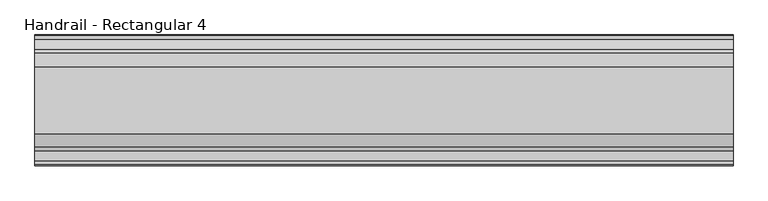
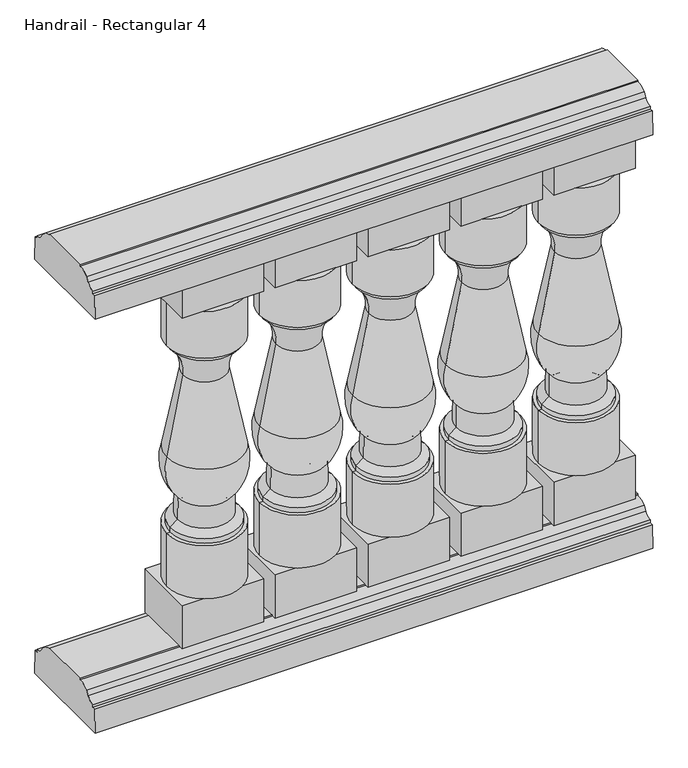
"""IFC4 building model written with IfcOpenShell, lengths in millimetres: railing geometry, Handrail - Rectangular 4."""

from ifc_helpers import new_model, si_unit, point, frame, frame_2d, origin, place, context, project, spatial, polyline, circle_curve, ellipse_curve, trimmed, segment, composite_curve, outline, extrude, source, transform, mapped, element, save
from ifc_brep_helpers import plane_surface, cylinder_surface, revolved_surface, advanced_brep


def handrail_rectangular_4_919d9a96(model_context):
    return source(origin(), model_context, "Body", "SolidModel", [
        extrude(outline(composite_curve([segment(trimmed(circle_curve(frame_2d((-1771.1852268, 1054.89375)), 19.84375), [point((-1771.1852268, 1035.05))], [point((-1754.064785, 1044.8605607))], True, "CARTESIAN"), True, "CONTINUOUS"), segment(polyline([(-1754.064785, 1044.8605607), (-1747.604713, 1054.3201059)]), True, "CONTINUOUS"), segment(trimmed(circle_curve(frame_2d((-1723.5602268, 1027.90625)), 35.71875), [point((-1747.604713, 1054.3201059))], [point((-1723.5602268, 1063.625))], False, "CARTESIAN"), True, "CONTINUOUS"), segment(polyline([(-1723.5602268, 1063.625), (-1723.5602268, 1066.8), (-1607.6727268, 1066.8), (-1607.6727268, 1063.625)]), True, "CONTINUOUS"), segment(trimmed(circle_curve(frame_2d((-1607.6727268, 1027.90625)), 35.71875), [point((-1607.6727268, 1063.625))], [point((-1583.6282406, 1054.3201059))], False, "CARTESIAN"), True, "CONTINUOUS"), segment(polyline([(-1583.6282406, 1054.3201059), (-1577.1681686, 1044.8605607)]), True, "CONTINUOUS"), segment(trimmed(circle_curve(frame_2d((-1560.0477268, 1054.89375)), 19.84375), [point((-1577.1681686, 1044.8605607))], [point((-1560.0477268, 1035.05))], True, "CARTESIAN"), True, "CONTINUOUS"), segment(polyline([(-1560.0477268, 1035.05), (-1560.0477268, 1028.7), (-1552.9039768, 1028.7), (-1551.3164768, 974.725), (-1779.9164768, 974.725), (-1778.3289768, 1028.7), (-1771.1852268, 1028.7), (-1771.1852268, 1035.05)]), True, "CONTINUOUS")], self_intersect=False)), frame((13827.6521895, 0.0, 0.0), z_axis=(1.0, 0.0, 0.0), x_axis=(0.0, 1.0, 0.0)), (0.0, 0.0, 1.0), 1219.2),
        extrude(outline(composite_curve([segment(trimmed(circle_curve(frame_2d((-1771.1852268, 99.21875)), 19.84375), [point((-1771.1852268, 79.375))], [point((-1754.064785, 89.1855607))], True, "CARTESIAN"), True, "CONTINUOUS"), segment(polyline([(-1754.064785, 89.1855607), (-1747.604713, 98.6451059)]), True, "CONTINUOUS"), segment(trimmed(circle_curve(frame_2d((-1723.5602268, 72.23125)), 35.71875), [point((-1747.604713, 98.6451059))], [point((-1723.5602268, 107.95))], False, "CARTESIAN"), True, "CONTINUOUS"), segment(polyline([(-1723.5602268, 107.95), (-1723.5602268, 111.125), (-1607.6727268, 111.125), (-1607.6727268, 107.95)]), True, "CONTINUOUS"), segment(trimmed(circle_curve(frame_2d((-1607.6727268, 72.23125)), 35.71875), [point((-1607.6727268, 107.95))], [point((-1583.6282406, 98.6451059))], False, "CARTESIAN"), True, "CONTINUOUS"), segment(polyline([(-1583.6282406, 98.6451059), (-1577.1681686, 89.1855607)]), True, "CONTINUOUS"), segment(trimmed(circle_curve(frame_2d((-1560.0477268, 99.21875)), 19.84375), [point((-1577.1681686, 89.1855607))], [point((-1560.0477268, 79.375))], True, "CARTESIAN"), True, "CONTINUOUS"), segment(polyline([(-1560.0477268, 79.375), (-1560.0477268, 73.025), (-1552.9039768, 73.025), (-1551.3164768, 19.05), (-1779.9164768, 19.05), (-1778.3289768, 73.025), (-1771.1852268, 73.025), (-1771.1852268, 79.375)]), True, "CONTINUOUS")], self_intersect=False)), frame((13827.6521895, 0.0, 0.0), z_axis=(1.0, 0.0, 0.0), x_axis=(0.0, 1.0, 0.0)), (0.0, 0.0, 1.0), 1219.2),
        advanced_brep(
        [(14862.7021895, -1665.6164768, 874.7125), (15027.8021895, -1665.6164768, 874.7125), (14945.2521895, -1665.6164768, 874.7125), (14862.7021895, -1665.6164768, 766.7625), (15027.8021895, -1665.6164768, 766.7625), (14870.6396895, -1665.6164768, 766.7625), (15019.8646895, -1665.6164768, 766.7625), (14870.6396895, -1665.6164768, 755.65), (15019.8646895, -1665.6164768, 755.65), (14898.4209395, -1665.6164768, 687.3875), (14992.0834395, -1665.6164768, 687.3875), (14863.4959395, -1665.6164768, 509.5875), (15027.0084395, -1665.6164768, 509.5875), (14887.3084395, -1665.6164768, 407.9875), (15003.1959395, -1665.6164768, 407.9875), (14886.5146895, -1665.6164768, 357.1875), (15003.9896895, -1665.6164768, 357.1875), (14870.6396895, -1665.6164768, 344.4875), (15019.8646895, -1665.6164768, 344.4875), (14870.6396895, -1665.6164768, 333.375), (15019.8646895, -1665.6164768, 333.375), (14862.7021895, -1665.6164768, 333.375), (15027.8021895, -1665.6164768, 333.375), (14862.7021895, -1665.6164768, 211.1375), (15027.8021895, -1665.6164768, 211.1375), (14945.2521895, -1665.6164768, 211.1375)],
        [
            (0, 1, circle_curve(frame((14945.2521895, -1665.6164768, 874.7125), z_axis=(0.0, 0.0, 1.0), x_axis=(1.0, 0.0, 0.0)), 82.55)),
            (1, 2),
            (2, 0),
            (1, 0, circle_curve(frame((14945.2521895, -1665.6164768, 874.7125), z_axis=(0.0, 0.0, 1.0), x_axis=(1.0, 0.0, 0.0)), 82.55)),
            (3, 4, circle_curve(frame((14945.2521895, -1665.6164768, 766.7625), z_axis=(0.0, 0.0, 1.0), x_axis=(1.0, 0.0, 0.0)), 82.55)),
            (4, 1),
            (0, 3),
            (4, 3, circle_curve(frame((14945.2521895, -1665.6164768, 766.7625), z_axis=(0.0, 0.0, 1.0), x_axis=(1.0, 0.0, 0.0)), 82.55)),
            (5, 6, circle_curve(frame((14945.2521895, -1665.6164768, 766.7625), z_axis=(0.0, 0.0, 1.0), x_axis=(1.0, 0.0, 0.0)), 74.6125)),
            (6, 4),
            (3, 5),
            (6, 5, circle_curve(frame((14945.2521895, -1665.6164768, 766.7625), z_axis=(0.0, 0.0, 1.0), x_axis=(1.0, 0.0, 0.0)), 74.6125)),
            (7, 8, circle_curve(frame((14945.2521895, -1665.6164768, 755.65), z_axis=(0.0, 0.0, 1.0), x_axis=(1.0, 0.0, 0.0)), 74.6125)),
            (8, 6),
            (5, 7),
            (8, 7, circle_curve(frame((14945.2521895, -1665.6164768, 755.65), z_axis=(0.0, 0.0, 1.0), x_axis=(1.0, 0.0, 0.0)), 74.6125)),
            (9, 10, circle_curve(frame((14945.2521895, -1665.6164768, 687.3875), z_axis=(0.0, 0.0, 1.0), x_axis=(1.0, 0.0, 0.0)), 46.83125)),
            (10, 8, circle_curve(frame((15071.2574242, -1665.6164768, 694.9499409), z_axis=(0.0, 1.0, 0.0), x_axis=(-1.0, 0.0, 0.0)), 79.5343344)),
            (7, 9, circle_curve(frame((14819.2469549, -1665.6164768, 694.9499409), z_axis=(0.0, 1.0, 0.0), x_axis=(1.0, 0.0, 0.0)), 79.5343344)),
            (10, 9, circle_curve(frame((14945.2521895, -1665.6164768, 687.3875), z_axis=(0.0, 0.0, 1.0), x_axis=(1.0, 0.0, 0.0)), 46.83125)),
            (11, 12, circle_curve(frame((14945.2521895, -1665.6164768, 509.5875), z_axis=(0.0, 0.0, 1.0), x_axis=(1.0, 0.0, 0.0)), 81.75625)),
            (12, 10, circle_curve(frame((15907.0418945, -1665.6164768, 774.7813483), z_axis=(0.0, 1.0, 0.0), x_axis=(-1.0, 0.0, 0.0)), 919.122766)),
            (9, 11, circle_curve(frame((13983.4624846, -1665.6164768, 774.7813483), z_axis=(0.0, 1.0, 0.0), x_axis=(1.0, 0.0, 0.0)), 919.122766)),
            (12, 11, circle_curve(frame((14945.2521895, -1665.6164768, 509.5875), z_axis=(0.0, 0.0, 1.0), x_axis=(1.0, 0.0, 0.0)), 81.75625)),
            (13, 14, circle_curve(frame((14945.2521895, -1665.6164768, 407.9875), z_axis=(0.0, 0.0, 1.0), x_axis=(1.0, 0.0, 0.0)), 57.94375)),
            (14, 12, circle_curve(frame((14926.9738909, -1665.6164768, 479.44257), z_axis=(0.0, -1.0, 0.0), x_axis=(-1.0, 0.0, 0.0)), 104.4778815)),
            (11, 13, circle_curve(frame((14963.5304882, -1665.6164768, 479.44257), z_axis=(0.0, -1.0, 0.0), x_axis=(1.0, 0.0, 0.0)), 104.4778815)),
            (14, 13, circle_curve(frame((14945.2521895, -1665.6164768, 407.9875), z_axis=(0.0, 0.0, 1.0), x_axis=(1.0, 0.0, 0.0)), 57.94375)),
            (15, 16, circle_curve(frame((14945.2521895, -1665.6164768, 357.1875), z_axis=(0.0, 0.0, 1.0), x_axis=(1.0, 0.0, 0.0)), 58.7375)),
            (16, 14),
            (13, 15),
            (16, 15, circle_curve(frame((14945.2521895, -1665.6164768, 357.1875), z_axis=(0.0, 0.0, 1.0), x_axis=(1.0, 0.0, 0.0)), 58.7375)),
            (17, 18, circle_curve(frame((14945.2521895, -1665.6164768, 344.4875), z_axis=(0.0, 0.0, 1.0), x_axis=(1.0, 0.0, 0.0)), 74.6125)),
            (18, 16),
            (15, 17),
            (18, 17, circle_curve(frame((14945.2521895, -1665.6164768, 344.4875), z_axis=(0.0, 0.0, 1.0), x_axis=(1.0, 0.0, 0.0)), 74.6125)),
            (19, 20, circle_curve(frame((14945.2521895, -1665.6164768, 333.375), z_axis=(0.0, 0.0, 1.0), x_axis=(1.0, 0.0, 0.0)), 74.6125)),
            (20, 18),
            (17, 19),
            (20, 19, circle_curve(frame((14945.2521895, -1665.6164768, 333.375), z_axis=(0.0, 0.0, 1.0), x_axis=(1.0, 0.0, 0.0)), 74.6125)),
            (21, 22, circle_curve(frame((14945.2521895, -1665.6164768, 333.375), z_axis=(0.0, 0.0, 1.0), x_axis=(1.0, 0.0, 0.0)), 82.55)),
            (22, 20),
            (19, 21),
            (22, 21, circle_curve(frame((14945.2521895, -1665.6164768, 333.375), z_axis=(0.0, 0.0, 1.0), x_axis=(1.0, 0.0, 0.0)), 82.55)),
            (23, 24, circle_curve(frame((14945.2521895, -1665.6164768, 211.1375), z_axis=(0.0, 0.0, 1.0), x_axis=(1.0, 0.0, 0.0)), 82.55)),
            (24, 22),
            (21, 23),
            (24, 23, circle_curve(frame((14945.2521895, -1665.6164768, 211.1375), z_axis=(0.0, 0.0, 1.0), x_axis=(1.0, 0.0, 0.0)), 82.55)),
            (25, 24),
            (23, 25),
        ],
        [
            plane_surface(frame((14945.2521895, -1665.6164768, 874.7125), z_axis=(0.0, 0.0, 1.0), x_axis=(1.0, 0.0, 0.0))),
            cylinder_surface(frame((14945.2521895, -1665.6164768, 839.7875), z_axis=(0.0, 0.0, -1.0), x_axis=(1.0, 0.0, 0.0)), 82.55),
            plane_surface(frame((14945.2521895, -1665.6164768, 766.7625), z_axis=(0.0, 0.0, -1.0), x_axis=(1.0, 0.0, 0.0))),
            cylinder_surface(frame((14945.2521895, -1665.6164768, 839.7875), z_axis=(0.0, 0.0, -1.0), x_axis=(1.0, 0.0, 0.0)), 74.6125),
            revolved_surface(trimmed(ellipse_curve(frame((15071.2574242, -1665.6164768, 694.9499409), z_axis=(0.0, -1.0, 0.0), x_axis=(-1.0, 0.0, 0.0)), 79.5343344, 79.5343344), [point((15019.8646895, -1665.6164768, 755.65))], [point((14992.0834395, -1665.6164768, 687.3875))], True, "CARTESIAN"), (14945.2521895, -1665.6164768, 839.7875), (0.0, 0.0, -1.0)),
            revolved_surface(trimmed(ellipse_curve(frame((15907.0418945, -1665.6164768, 774.7813483), z_axis=(0.0, -1.0, 0.0), x_axis=(-1.0, 0.0, 0.0)), 919.122766, 919.122766), [point((14992.0834395, -1665.6164768, 687.3875))], [point((15027.0084395, -1665.6164768, 509.5875))], True, "CARTESIAN"), (14945.2521895, -1665.6164768, 839.7875), (0.0, 0.0, -1.0)),
            revolved_surface(trimmed(ellipse_curve(frame((14926.9738909, -1665.6164768, 479.44257), z_axis=(0.0, 1.0, 0.0), x_axis=(-1.0, 0.0, 0.0)), 104.4778815, 104.4778815), [point((15027.0084395, -1665.6164768, 509.5875))], [point((15003.1959395, -1665.6164768, 407.9875))], True, "CARTESIAN"), (14945.2521895, -1665.6164768, 839.7875), (0.0, 0.0, -1.0)),
            revolved_surface(polyline([(15003.1959395, -1665.6164768, 407.9875), (15003.9896895, -1665.6164768, 357.1875)]), (14945.2521895, -1665.6164768, 839.7875), (0.0, 0.0, -1.0)),
            revolved_surface(polyline([(15003.9896895, -1665.6164768, 357.1875), (15019.8646895, -1665.6164768, 344.4875)]), (14945.2521895, -1665.6164768, 839.7875), (0.0, 0.0, -1.0)),
            plane_surface(frame((14945.2521895, -1665.6164768, 333.375), z_axis=(0.0, 0.0, 1.0), x_axis=(1.0, 0.0, 0.0))),
            plane_surface(frame((14945.2521895, -1665.6164768, 211.1375), z_axis=(0.0, 0.0, -1.0), x_axis=(1.0, 0.0, 0.0))),
        ],
        [
            (0, [[1, 2, 3]]),
            (0, [[4, -3, -2]]),
            (1, [[5, 6, -1, 7]]),
            (1, [[8, -7, -4, -6]]),
            (2, [[9, 10, -5, 11]]),
            (2, [[12, -11, -8, -10]]),
            (3, [[13, 14, -9, 15]]),
            (3, [[16, -15, -12, -14]]),
            (4, [[17, 18, -13, 19]]),
            (4, [[20, -19, -16, -18]]),
            (5, [[21, 22, -17, 23]]),
            (5, [[24, -23, -20, -22]]),
            (6, [[25, 26, -21, 27]]),
            (6, [[28, -27, -24, -26]]),
            (7, [[29, 30, -25, 31]]),
            (7, [[32, -31, -28, -30]]),
            (8, [[33, 34, -29, 35]]),
            (8, [[36, -35, -32, -34]]),
            (3, [[37, 38, -33, 39]]),
            (3, [[40, -39, -36, -38]]),
            (9, [[41, 42, -37, 43]]),
            (9, [[44, -43, -40, -42]]),
            (1, [[45, 46, -41, 47]]),
            (1, [[48, -47, -44, -46]]),
            (10, [[49, -45, 50]]),
            (10, [[-50, -48, -49]]),
        ],
    ),
        extrude(outline(polyline([(14856.3521895, -1735.4664768), (14856.3521895, -1595.7664768), (15034.1521895, -1595.7664768), (15034.1521895, -1735.4664768), (14856.3521895, -1735.4664768)])), frame((0.0, 0.0, 111.125), z_axis=(0.0, 0.0, 1.0), x_axis=(1.0, 0.0, 0.0)), (0.0, 0.0, 1.0), 100.0125),
        extrude(outline(polyline([(14856.3521895, -1595.7664768), (15034.1521895, -1595.7664768), (15034.1521895, -1735.4664768), (14856.3521895, -1735.4664768), (14856.3521895, -1595.7664768)])), frame((0.0, 0.0, 874.7125), z_axis=(0.0, 0.0, 1.0), x_axis=(1.0, 0.0, 0.0)), (0.0, 0.0, 1.0), 100.0125),
        advanced_brep(
        [(14659.5021895, -1665.6164768, 874.7125), (14824.6021895, -1665.6164768, 874.7125), (14742.0521895, -1665.6164768, 874.7125), (14659.5021895, -1665.6164768, 766.7625), (14824.6021895, -1665.6164768, 766.7625), (14667.4396895, -1665.6164768, 766.7625), (14816.6646895, -1665.6164768, 766.7625), (14667.4396895, -1665.6164768, 755.65), (14816.6646895, -1665.6164768, 755.65), (14695.2209395, -1665.6164768, 687.3875), (14788.8834395, -1665.6164768, 687.3875), (14660.2959395, -1665.6164768, 509.5875), (14823.8084395, -1665.6164768, 509.5875), (14684.1084395, -1665.6164768, 407.9875), (14799.9959395, -1665.6164768, 407.9875), (14683.3146895, -1665.6164768, 357.1875), (14800.7896895, -1665.6164768, 357.1875), (14667.4396895, -1665.6164768, 344.4875), (14816.6646895, -1665.6164768, 344.4875), (14667.4396895, -1665.6164768, 333.375), (14816.6646895, -1665.6164768, 333.375), (14659.5021895, -1665.6164768, 333.375), (14824.6021895, -1665.6164768, 333.375), (14659.5021895, -1665.6164768, 211.1375), (14824.6021895, -1665.6164768, 211.1375), (14742.0521895, -1665.6164768, 211.1375)],
        [
            (0, 1, circle_curve(frame((14742.0521895, -1665.6164768, 874.7125), z_axis=(0.0, 0.0, 1.0), x_axis=(1.0, 0.0, 0.0)), 82.55)),
            (1, 2),
            (2, 0),
            (1, 0, circle_curve(frame((14742.0521895, -1665.6164768, 874.7125), z_axis=(0.0, 0.0, 1.0), x_axis=(1.0, 0.0, 0.0)), 82.55)),
            (3, 4, circle_curve(frame((14742.0521895, -1665.6164768, 766.7625), z_axis=(0.0, 0.0, 1.0), x_axis=(1.0, 0.0, 0.0)), 82.55)),
            (4, 1),
            (0, 3),
            (4, 3, circle_curve(frame((14742.0521895, -1665.6164768, 766.7625), z_axis=(0.0, 0.0, 1.0), x_axis=(1.0, 0.0, 0.0)), 82.55)),
            (5, 6, circle_curve(frame((14742.0521895, -1665.6164768, 766.7625), z_axis=(0.0, 0.0, 1.0), x_axis=(1.0, 0.0, 0.0)), 74.6125)),
            (6, 4),
            (3, 5),
            (6, 5, circle_curve(frame((14742.0521895, -1665.6164768, 766.7625), z_axis=(0.0, 0.0, 1.0), x_axis=(1.0, 0.0, 0.0)), 74.6125)),
            (7, 8, circle_curve(frame((14742.0521895, -1665.6164768, 755.65), z_axis=(0.0, 0.0, 1.0), x_axis=(1.0, 0.0, 0.0)), 74.6125)),
            (8, 6),
            (5, 7),
            (8, 7, circle_curve(frame((14742.0521895, -1665.6164768, 755.65), z_axis=(0.0, 0.0, 1.0), x_axis=(1.0, 0.0, 0.0)), 74.6125)),
            (9, 10, circle_curve(frame((14742.0521895, -1665.6164768, 687.3875), z_axis=(0.0, 0.0, 1.0), x_axis=(1.0, 0.0, 0.0)), 46.83125)),
            (10, 8, circle_curve(frame((14868.0574242, -1665.6164768, 694.9499409), z_axis=(0.0, 1.0, 0.0), x_axis=(-1.0, 0.0, 0.0)), 79.5343344)),
            (7, 9, circle_curve(frame((14616.0469549, -1665.6164768, 694.9499409), z_axis=(0.0, 1.0, 0.0), x_axis=(1.0, 0.0, 0.0)), 79.5343344)),
            (10, 9, circle_curve(frame((14742.0521895, -1665.6164768, 687.3875), z_axis=(0.0, 0.0, 1.0), x_axis=(1.0, 0.0, 0.0)), 46.83125)),
            (11, 12, circle_curve(frame((14742.0521895, -1665.6164768, 509.5875), z_axis=(0.0, 0.0, 1.0), x_axis=(1.0, 0.0, 0.0)), 81.75625)),
            (12, 10, circle_curve(frame((15703.8418945, -1665.6164768, 774.7813483), z_axis=(0.0, 1.0, 0.0), x_axis=(-1.0, 0.0, 0.0)), 919.122766)),
            (9, 11, circle_curve(frame((13780.2624846, -1665.6164768, 774.7813483), z_axis=(0.0, 1.0, 0.0), x_axis=(1.0, 0.0, 0.0)), 919.122766)),
            (12, 11, circle_curve(frame((14742.0521895, -1665.6164768, 509.5875), z_axis=(0.0, 0.0, 1.0), x_axis=(1.0, 0.0, 0.0)), 81.75625)),
            (13, 14, circle_curve(frame((14742.0521895, -1665.6164768, 407.9875), z_axis=(0.0, 0.0, 1.0), x_axis=(1.0, 0.0, 0.0)), 57.94375)),
            (14, 12, circle_curve(frame((14723.7738909, -1665.6164768, 479.44257), z_axis=(0.0, -1.0, 0.0), x_axis=(-1.0, 0.0, 0.0)), 104.4778815)),
            (11, 13, circle_curve(frame((14760.3304882, -1665.6164768, 479.44257), z_axis=(0.0, -1.0, 0.0), x_axis=(1.0, 0.0, 0.0)), 104.4778815)),
            (14, 13, circle_curve(frame((14742.0521895, -1665.6164768, 407.9875), z_axis=(0.0, 0.0, 1.0), x_axis=(1.0, 0.0, 0.0)), 57.94375)),
            (15, 16, circle_curve(frame((14742.0521895, -1665.6164768, 357.1875), z_axis=(0.0, 0.0, 1.0), x_axis=(1.0, 0.0, 0.0)), 58.7375)),
            (16, 14),
            (13, 15),
            (16, 15, circle_curve(frame((14742.0521895, -1665.6164768, 357.1875), z_axis=(0.0, 0.0, 1.0), x_axis=(1.0, 0.0, 0.0)), 58.7375)),
            (17, 18, circle_curve(frame((14742.0521895, -1665.6164768, 344.4875), z_axis=(0.0, 0.0, 1.0), x_axis=(1.0, 0.0, 0.0)), 74.6125)),
            (18, 16),
            (15, 17),
            (18, 17, circle_curve(frame((14742.0521895, -1665.6164768, 344.4875), z_axis=(0.0, 0.0, 1.0), x_axis=(1.0, 0.0, 0.0)), 74.6125)),
            (19, 20, circle_curve(frame((14742.0521895, -1665.6164768, 333.375), z_axis=(0.0, 0.0, 1.0), x_axis=(1.0, 0.0, 0.0)), 74.6125)),
            (20, 18),
            (17, 19),
            (20, 19, circle_curve(frame((14742.0521895, -1665.6164768, 333.375), z_axis=(0.0, 0.0, 1.0), x_axis=(1.0, 0.0, 0.0)), 74.6125)),
            (21, 22, circle_curve(frame((14742.0521895, -1665.6164768, 333.375), z_axis=(0.0, 0.0, 1.0), x_axis=(1.0, 0.0, 0.0)), 82.55)),
            (22, 20),
            (19, 21),
            (22, 21, circle_curve(frame((14742.0521895, -1665.6164768, 333.375), z_axis=(0.0, 0.0, 1.0), x_axis=(1.0, 0.0, 0.0)), 82.55)),
            (23, 24, circle_curve(frame((14742.0521895, -1665.6164768, 211.1375), z_axis=(0.0, 0.0, 1.0), x_axis=(1.0, 0.0, 0.0)), 82.55)),
            (24, 22),
            (21, 23),
            (24, 23, circle_curve(frame((14742.0521895, -1665.6164768, 211.1375), z_axis=(0.0, 0.0, 1.0), x_axis=(1.0, 0.0, 0.0)), 82.55)),
            (25, 24),
            (23, 25),
        ],
        [
            plane_surface(frame((14742.0521895, -1665.6164768, 874.7125), z_axis=(0.0, 0.0, 1.0), x_axis=(1.0, 0.0, 0.0))),
            cylinder_surface(frame((14742.0521895, -1665.6164768, 839.7875), z_axis=(0.0, 0.0, -1.0), x_axis=(1.0, 0.0, 0.0)), 82.55),
            plane_surface(frame((14742.0521895, -1665.6164768, 766.7625), z_axis=(0.0, 0.0, -1.0), x_axis=(1.0, 0.0, 0.0))),
            cylinder_surface(frame((14742.0521895, -1665.6164768, 839.7875), z_axis=(0.0, 0.0, -1.0), x_axis=(1.0, 0.0, 0.0)), 74.6125),
            revolved_surface(trimmed(ellipse_curve(frame((14868.0574242, -1665.6164768, 694.9499409), z_axis=(0.0, -1.0, 0.0), x_axis=(-1.0, 0.0, 0.0)), 79.5343344, 79.5343344), [point((14816.6646895, -1665.6164768, 755.65))], [point((14788.8834395, -1665.6164768, 687.3875))], True, "CARTESIAN"), (14742.0521895, -1665.6164768, 839.7875), (0.0, 0.0, -1.0)),
            revolved_surface(trimmed(ellipse_curve(frame((15703.8418945, -1665.6164768, 774.7813483), z_axis=(0.0, -1.0, 0.0), x_axis=(-1.0, 0.0, 0.0)), 919.122766, 919.122766), [point((14788.8834395, -1665.6164768, 687.3875))], [point((14823.8084395, -1665.6164768, 509.5875))], True, "CARTESIAN"), (14742.0521895, -1665.6164768, 839.7875), (0.0, 0.0, -1.0)),
            revolved_surface(trimmed(ellipse_curve(frame((14723.7738909, -1665.6164768, 479.44257), z_axis=(0.0, 1.0, 0.0), x_axis=(-1.0, 0.0, 0.0)), 104.4778815, 104.4778815), [point((14823.8084395, -1665.6164768, 509.5875))], [point((14799.9959395, -1665.6164768, 407.9875))], True, "CARTESIAN"), (14742.0521895, -1665.6164768, 839.7875), (0.0, 0.0, -1.0)),
            revolved_surface(polyline([(14799.9959395, -1665.6164768, 407.9875), (14800.7896895, -1665.6164768, 357.1875)]), (14742.0521895, -1665.6164768, 839.7875), (0.0, 0.0, -1.0)),
            revolved_surface(polyline([(14800.7896895, -1665.6164768, 357.1875), (14816.6646895, -1665.6164768, 344.4875)]), (14742.0521895, -1665.6164768, 839.7875), (0.0, 0.0, -1.0)),
            plane_surface(frame((14742.0521895, -1665.6164768, 333.375), z_axis=(0.0, 0.0, 1.0), x_axis=(1.0, 0.0, 0.0))),
            plane_surface(frame((14742.0521895, -1665.6164768, 211.1375), z_axis=(0.0, 0.0, -1.0), x_axis=(1.0, 0.0, 0.0))),
        ],
        [
            (0, [[1, 2, 3]]),
            (0, [[4, -3, -2]]),
            (1, [[5, 6, -1, 7]]),
            (1, [[8, -7, -4, -6]]),
            (2, [[9, 10, -5, 11]]),
            (2, [[12, -11, -8, -10]]),
            (3, [[13, 14, -9, 15]]),
            (3, [[16, -15, -12, -14]]),
            (4, [[17, 18, -13, 19]]),
            (4, [[20, -19, -16, -18]]),
            (5, [[21, 22, -17, 23]]),
            (5, [[24, -23, -20, -22]]),
            (6, [[25, 26, -21, 27]]),
            (6, [[28, -27, -24, -26]]),
            (7, [[29, 30, -25, 31]]),
            (7, [[32, -31, -28, -30]]),
            (8, [[33, 34, -29, 35]]),
            (8, [[36, -35, -32, -34]]),
            (3, [[37, 38, -33, 39]]),
            (3, [[40, -39, -36, -38]]),
            (9, [[41, 42, -37, 43]]),
            (9, [[44, -43, -40, -42]]),
            (1, [[45, 46, -41, 47]]),
            (1, [[48, -47, -44, -46]]),
            (10, [[49, -45, 50]]),
            (10, [[-50, -48, -49]]),
        ],
    ),
        extrude(outline(polyline([(14653.1521895, -1735.4664768), (14653.1521895, -1595.7664768), (14830.9521895, -1595.7664768), (14830.9521895, -1735.4664768), (14653.1521895, -1735.4664768)])), frame((0.0, 0.0, 111.125), z_axis=(0.0, 0.0, 1.0), x_axis=(1.0, 0.0, 0.0)), (0.0, 0.0, 1.0), 100.0125),
        extrude(outline(polyline([(14653.1521895, -1595.7664768), (14830.9521895, -1595.7664768), (14830.9521895, -1735.4664768), (14653.1521895, -1735.4664768), (14653.1521895, -1595.7664768)])), frame((0.0, 0.0, 874.7125), z_axis=(0.0, 0.0, 1.0), x_axis=(1.0, 0.0, 0.0)), (0.0, 0.0, 1.0), 100.0125),
        advanced_brep(
        [(14456.3021895, -1665.6164768, 874.7125), (14621.4021895, -1665.6164768, 874.7125), (14538.8521895, -1665.6164768, 874.7125), (14456.3021895, -1665.6164768, 766.7625), (14621.4021895, -1665.6164768, 766.7625), (14464.2396895, -1665.6164768, 766.7625), (14613.4646895, -1665.6164768, 766.7625), (14464.2396895, -1665.6164768, 755.65), (14613.4646895, -1665.6164768, 755.65), (14492.0209395, -1665.6164768, 687.3875), (14585.6834395, -1665.6164768, 687.3875), (14457.0959395, -1665.6164768, 509.5875), (14620.6084395, -1665.6164768, 509.5875), (14480.9084395, -1665.6164768, 407.9875), (14596.7959395, -1665.6164768, 407.9875), (14480.1146895, -1665.6164768, 357.1875), (14597.5896895, -1665.6164768, 357.1875), (14464.2396895, -1665.6164768, 344.4875), (14613.4646895, -1665.6164768, 344.4875), (14464.2396895, -1665.6164768, 333.375), (14613.4646895, -1665.6164768, 333.375), (14456.3021895, -1665.6164768, 333.375), (14621.4021895, -1665.6164768, 333.375), (14456.3021895, -1665.6164768, 211.1375), (14621.4021895, -1665.6164768, 211.1375), (14538.8521895, -1665.6164768, 211.1375)],
        [
            (0, 1, circle_curve(frame((14538.8521895, -1665.6164768, 874.7125), z_axis=(0.0, 0.0, 1.0), x_axis=(1.0, 0.0, 0.0)), 82.55)),
            (1, 2),
            (2, 0),
            (1, 0, circle_curve(frame((14538.8521895, -1665.6164768, 874.7125), z_axis=(0.0, 0.0, 1.0), x_axis=(1.0, 0.0, 0.0)), 82.55)),
            (3, 4, circle_curve(frame((14538.8521895, -1665.6164768, 766.7625), z_axis=(0.0, 0.0, 1.0), x_axis=(1.0, 0.0, 0.0)), 82.55)),
            (4, 1),
            (0, 3),
            (4, 3, circle_curve(frame((14538.8521895, -1665.6164768, 766.7625), z_axis=(0.0, 0.0, 1.0), x_axis=(1.0, 0.0, 0.0)), 82.55)),
            (5, 6, circle_curve(frame((14538.8521895, -1665.6164768, 766.7625), z_axis=(0.0, 0.0, 1.0), x_axis=(1.0, 0.0, 0.0)), 74.6125)),
            (6, 4),
            (3, 5),
            (6, 5, circle_curve(frame((14538.8521895, -1665.6164768, 766.7625), z_axis=(0.0, 0.0, 1.0), x_axis=(1.0, 0.0, 0.0)), 74.6125)),
            (7, 8, circle_curve(frame((14538.8521895, -1665.6164768, 755.65), z_axis=(0.0, 0.0, 1.0), x_axis=(1.0, 0.0, 0.0)), 74.6125)),
            (8, 6),
            (5, 7),
            (8, 7, circle_curve(frame((14538.8521895, -1665.6164768, 755.65), z_axis=(0.0, 0.0, 1.0), x_axis=(1.0, 0.0, 0.0)), 74.6125)),
            (9, 10, circle_curve(frame((14538.8521895, -1665.6164768, 687.3875), z_axis=(0.0, 0.0, 1.0), x_axis=(1.0, 0.0, 0.0)), 46.83125)),
            (10, 8, circle_curve(frame((14664.8574242, -1665.6164768, 694.9499409), z_axis=(0.0, 1.0, 0.0), x_axis=(-1.0, 0.0, 0.0)), 79.5343344)),
            (7, 9, circle_curve(frame((14412.8469549, -1665.6164768, 694.9499409), z_axis=(0.0, 1.0, 0.0), x_axis=(1.0, 0.0, 0.0)), 79.5343344)),
            (10, 9, circle_curve(frame((14538.8521895, -1665.6164768, 687.3875), z_axis=(0.0, 0.0, 1.0), x_axis=(1.0, 0.0, 0.0)), 46.83125)),
            (11, 12, circle_curve(frame((14538.8521895, -1665.6164768, 509.5875), z_axis=(0.0, 0.0, 1.0), x_axis=(1.0, 0.0, 0.0)), 81.75625)),
            (12, 10, circle_curve(frame((15500.6418945, -1665.6164768, 774.7813483), z_axis=(0.0, 1.0, 0.0), x_axis=(-1.0, 0.0, 0.0)), 919.122766)),
            (9, 11, circle_curve(frame((13577.0624846, -1665.6164768, 774.7813483), z_axis=(0.0, 1.0, 0.0), x_axis=(1.0, 0.0, 0.0)), 919.122766)),
            (12, 11, circle_curve(frame((14538.8521895, -1665.6164768, 509.5875), z_axis=(0.0, 0.0, 1.0), x_axis=(1.0, 0.0, 0.0)), 81.75625)),
            (13, 14, circle_curve(frame((14538.8521895, -1665.6164768, 407.9875), z_axis=(0.0, 0.0, 1.0), x_axis=(1.0, 0.0, 0.0)), 57.94375)),
            (14, 12, circle_curve(frame((14520.5738909, -1665.6164768, 479.44257), z_axis=(0.0, -1.0, 0.0), x_axis=(-1.0, 0.0, 0.0)), 104.4778815)),
            (11, 13, circle_curve(frame((14557.1304882, -1665.6164768, 479.44257), z_axis=(0.0, -1.0, 0.0), x_axis=(1.0, 0.0, 0.0)), 104.4778815)),
            (14, 13, circle_curve(frame((14538.8521895, -1665.6164768, 407.9875), z_axis=(0.0, 0.0, 1.0), x_axis=(1.0, 0.0, 0.0)), 57.94375)),
            (15, 16, circle_curve(frame((14538.8521895, -1665.6164768, 357.1875), z_axis=(0.0, 0.0, 1.0), x_axis=(1.0, 0.0, 0.0)), 58.7375)),
            (16, 14),
            (13, 15),
            (16, 15, circle_curve(frame((14538.8521895, -1665.6164768, 357.1875), z_axis=(0.0, 0.0, 1.0), x_axis=(1.0, 0.0, 0.0)), 58.7375)),
            (17, 18, circle_curve(frame((14538.8521895, -1665.6164768, 344.4875), z_axis=(0.0, 0.0, 1.0), x_axis=(1.0, 0.0, 0.0)), 74.6125)),
            (18, 16),
            (15, 17),
            (18, 17, circle_curve(frame((14538.8521895, -1665.6164768, 344.4875), z_axis=(0.0, 0.0, 1.0), x_axis=(1.0, 0.0, 0.0)), 74.6125)),
            (19, 20, circle_curve(frame((14538.8521895, -1665.6164768, 333.375), z_axis=(0.0, 0.0, 1.0), x_axis=(1.0, 0.0, 0.0)), 74.6125)),
            (20, 18),
            (17, 19),
            (20, 19, circle_curve(frame((14538.8521895, -1665.6164768, 333.375), z_axis=(0.0, 0.0, 1.0), x_axis=(1.0, 0.0, 0.0)), 74.6125)),
            (21, 22, circle_curve(frame((14538.8521895, -1665.6164768, 333.375), z_axis=(0.0, 0.0, 1.0), x_axis=(1.0, 0.0, 0.0)), 82.55)),
            (22, 20),
            (19, 21),
            (22, 21, circle_curve(frame((14538.8521895, -1665.6164768, 333.375), z_axis=(0.0, 0.0, 1.0), x_axis=(1.0, 0.0, 0.0)), 82.55)),
            (23, 24, circle_curve(frame((14538.8521895, -1665.6164768, 211.1375), z_axis=(0.0, 0.0, 1.0), x_axis=(1.0, 0.0, 0.0)), 82.55)),
            (24, 22),
            (21, 23),
            (24, 23, circle_curve(frame((14538.8521895, -1665.6164768, 211.1375), z_axis=(0.0, 0.0, 1.0), x_axis=(1.0, 0.0, 0.0)), 82.55)),
            (25, 24),
            (23, 25),
        ],
        [
            plane_surface(frame((14538.8521895, -1665.6164768, 874.7125), z_axis=(0.0, 0.0, 1.0), x_axis=(1.0, 0.0, 0.0))),
            cylinder_surface(frame((14538.8521895, -1665.6164768, 839.7875), z_axis=(0.0, 0.0, -1.0), x_axis=(1.0, 0.0, 0.0)), 82.55),
            plane_surface(frame((14538.8521895, -1665.6164768, 766.7625), z_axis=(0.0, 0.0, -1.0), x_axis=(1.0, 0.0, 0.0))),
            cylinder_surface(frame((14538.8521895, -1665.6164768, 839.7875), z_axis=(0.0, 0.0, -1.0), x_axis=(1.0, 0.0, 0.0)), 74.6125),
            revolved_surface(trimmed(ellipse_curve(frame((14664.8574242, -1665.6164768, 694.9499409), z_axis=(0.0, -1.0, 0.0), x_axis=(-1.0, 0.0, 0.0)), 79.5343344, 79.5343344), [point((14613.4646895, -1665.6164768, 755.65))], [point((14585.6834395, -1665.6164768, 687.3875))], True, "CARTESIAN"), (14538.8521895, -1665.6164768, 839.7875), (0.0, 0.0, -1.0)),
            revolved_surface(trimmed(ellipse_curve(frame((15500.6418945, -1665.6164768, 774.7813483), z_axis=(0.0, -1.0, 0.0), x_axis=(-1.0, 0.0, 0.0)), 919.122766, 919.122766), [point((14585.6834395, -1665.6164768, 687.3875))], [point((14620.6084395, -1665.6164768, 509.5875))], True, "CARTESIAN"), (14538.8521895, -1665.6164768, 839.7875), (0.0, 0.0, -1.0)),
            revolved_surface(trimmed(ellipse_curve(frame((14520.5738909, -1665.6164768, 479.44257), z_axis=(0.0, 1.0, 0.0), x_axis=(-1.0, 0.0, 0.0)), 104.4778815, 104.4778815), [point((14620.6084395, -1665.6164768, 509.5875))], [point((14596.7959395, -1665.6164768, 407.9875))], True, "CARTESIAN"), (14538.8521895, -1665.6164768, 839.7875), (0.0, 0.0, -1.0)),
            revolved_surface(polyline([(14596.7959395, -1665.6164768, 407.9875), (14597.5896895, -1665.6164768, 357.1875)]), (14538.8521895, -1665.6164768, 839.7875), (0.0, 0.0, -1.0)),
            revolved_surface(polyline([(14597.5896895, -1665.6164768, 357.1875), (14613.4646895, -1665.6164768, 344.4875)]), (14538.8521895, -1665.6164768, 839.7875), (0.0, 0.0, -1.0)),
            plane_surface(frame((14538.8521895, -1665.6164768, 333.375), z_axis=(0.0, 0.0, 1.0), x_axis=(1.0, 0.0, 0.0))),
            plane_surface(frame((14538.8521895, -1665.6164768, 211.1375), z_axis=(0.0, 0.0, -1.0), x_axis=(1.0, 0.0, 0.0))),
        ],
        [
            (0, [[1, 2, 3]]),
            (0, [[4, -3, -2]]),
            (1, [[5, 6, -1, 7]]),
            (1, [[8, -7, -4, -6]]),
            (2, [[9, 10, -5, 11]]),
            (2, [[12, -11, -8, -10]]),
            (3, [[13, 14, -9, 15]]),
            (3, [[16, -15, -12, -14]]),
            (4, [[17, 18, -13, 19]]),
            (4, [[20, -19, -16, -18]]),
            (5, [[21, 22, -17, 23]]),
            (5, [[24, -23, -20, -22]]),
            (6, [[25, 26, -21, 27]]),
            (6, [[28, -27, -24, -26]]),
            (7, [[29, 30, -25, 31]]),
            (7, [[32, -31, -28, -30]]),
            (8, [[33, 34, -29, 35]]),
            (8, [[36, -35, -32, -34]]),
            (3, [[37, 38, -33, 39]]),
            (3, [[40, -39, -36, -38]]),
            (9, [[41, 42, -37, 43]]),
            (9, [[44, -43, -40, -42]]),
            (1, [[45, 46, -41, 47]]),
            (1, [[48, -47, -44, -46]]),
            (10, [[49, -45, 50]]),
            (10, [[-50, -48, -49]]),
        ],
    ),
        extrude(outline(polyline([(14449.9521895, -1735.4664768), (14449.9521895, -1595.7664768), (14627.7521895, -1595.7664768), (14627.7521895, -1735.4664768), (14449.9521895, -1735.4664768)])), frame((0.0, 0.0, 111.125), z_axis=(0.0, 0.0, 1.0), x_axis=(1.0, 0.0, 0.0)), (0.0, 0.0, 1.0), 100.0125),
        extrude(outline(polyline([(14449.9521895, -1595.7664768), (14627.7521895, -1595.7664768), (14627.7521895, -1735.4664768), (14449.9521895, -1735.4664768), (14449.9521895, -1595.7664768)])), frame((0.0, 0.0, 874.7125), z_axis=(0.0, 0.0, 1.0), x_axis=(1.0, 0.0, 0.0)), (0.0, 0.0, 1.0), 100.0125),
        advanced_brep(
        [(14253.1021895, -1665.6164768, 874.7125), (14418.2021895, -1665.6164768, 874.7125), (14335.6521895, -1665.6164768, 874.7125), (14253.1021895, -1665.6164768, 766.7625), (14418.2021895, -1665.6164768, 766.7625), (14261.0396895, -1665.6164768, 766.7625), (14410.2646895, -1665.6164768, 766.7625), (14261.0396895, -1665.6164768, 755.65), (14410.2646895, -1665.6164768, 755.65), (14288.8209395, -1665.6164768, 687.3875), (14382.4834395, -1665.6164768, 687.3875), (14253.8959395, -1665.6164768, 509.5875), (14417.4084395, -1665.6164768, 509.5875), (14277.7084395, -1665.6164768, 407.9875), (14393.5959395, -1665.6164768, 407.9875), (14276.9146895, -1665.6164768, 357.1875), (14394.3896895, -1665.6164768, 357.1875), (14261.0396895, -1665.6164768, 344.4875), (14410.2646895, -1665.6164768, 344.4875), (14261.0396895, -1665.6164768, 333.375), (14410.2646895, -1665.6164768, 333.375), (14253.1021895, -1665.6164768, 333.375), (14418.2021895, -1665.6164768, 333.375), (14253.1021895, -1665.6164768, 211.1375), (14418.2021895, -1665.6164768, 211.1375), (14335.6521895, -1665.6164768, 211.1375)],
        [
            (0, 1, circle_curve(frame((14335.6521895, -1665.6164768, 874.7125), z_axis=(0.0, 0.0, 1.0), x_axis=(1.0, 0.0, 0.0)), 82.55)),
            (1, 2),
            (2, 0),
            (1, 0, circle_curve(frame((14335.6521895, -1665.6164768, 874.7125), z_axis=(0.0, 0.0, 1.0), x_axis=(1.0, 0.0, 0.0)), 82.55)),
            (3, 4, circle_curve(frame((14335.6521895, -1665.6164768, 766.7625), z_axis=(0.0, 0.0, 1.0), x_axis=(1.0, 0.0, 0.0)), 82.55)),
            (4, 1),
            (0, 3),
            (4, 3, circle_curve(frame((14335.6521895, -1665.6164768, 766.7625), z_axis=(0.0, 0.0, 1.0), x_axis=(1.0, 0.0, 0.0)), 82.55)),
            (5, 6, circle_curve(frame((14335.6521895, -1665.6164768, 766.7625), z_axis=(0.0, 0.0, 1.0), x_axis=(1.0, 0.0, 0.0)), 74.6125)),
            (6, 4),
            (3, 5),
            (6, 5, circle_curve(frame((14335.6521895, -1665.6164768, 766.7625), z_axis=(0.0, 0.0, 1.0), x_axis=(1.0, 0.0, 0.0)), 74.6125)),
            (7, 8, circle_curve(frame((14335.6521895, -1665.6164768, 755.65), z_axis=(0.0, 0.0, 1.0), x_axis=(1.0, 0.0, 0.0)), 74.6125)),
            (8, 6),
            (5, 7),
            (8, 7, circle_curve(frame((14335.6521895, -1665.6164768, 755.65), z_axis=(0.0, 0.0, 1.0), x_axis=(1.0, 0.0, 0.0)), 74.6125)),
            (9, 10, circle_curve(frame((14335.6521895, -1665.6164768, 687.3875), z_axis=(0.0, 0.0, 1.0), x_axis=(1.0, 0.0, 0.0)), 46.83125)),
            (10, 8, circle_curve(frame((14461.6574242, -1665.6164768, 694.9499409), z_axis=(0.0, 1.0, 0.0), x_axis=(-1.0, 0.0, 0.0)), 79.5343344)),
            (7, 9, circle_curve(frame((14209.6469549, -1665.6164768, 694.9499409), z_axis=(0.0, 1.0, 0.0), x_axis=(1.0, 0.0, 0.0)), 79.5343344)),
            (10, 9, circle_curve(frame((14335.6521895, -1665.6164768, 687.3875), z_axis=(0.0, 0.0, 1.0), x_axis=(1.0, 0.0, 0.0)), 46.83125)),
            (11, 12, circle_curve(frame((14335.6521895, -1665.6164768, 509.5875), z_axis=(0.0, 0.0, 1.0), x_axis=(1.0, 0.0, 0.0)), 81.75625)),
            (12, 10, circle_curve(frame((15297.4418945, -1665.6164768, 774.7813483), z_axis=(0.0, 1.0, 0.0), x_axis=(-1.0, 0.0, 0.0)), 919.122766)),
            (9, 11, circle_curve(frame((13373.8624846, -1665.6164768, 774.7813483), z_axis=(0.0, 1.0, 0.0), x_axis=(1.0, 0.0, 0.0)), 919.122766)),
            (12, 11, circle_curve(frame((14335.6521895, -1665.6164768, 509.5875), z_axis=(0.0, 0.0, 1.0), x_axis=(1.0, 0.0, 0.0)), 81.75625)),
            (13, 14, circle_curve(frame((14335.6521895, -1665.6164768, 407.9875), z_axis=(0.0, 0.0, 1.0), x_axis=(1.0, 0.0, 0.0)), 57.94375)),
            (14, 12, circle_curve(frame((14317.3738909, -1665.6164768, 479.44257), z_axis=(0.0, -1.0, 0.0), x_axis=(-1.0, 0.0, 0.0)), 104.4778815)),
            (11, 13, circle_curve(frame((14353.9304882, -1665.6164768, 479.44257), z_axis=(0.0, -1.0, 0.0), x_axis=(1.0, 0.0, 0.0)), 104.4778815)),
            (14, 13, circle_curve(frame((14335.6521895, -1665.6164768, 407.9875), z_axis=(0.0, 0.0, 1.0), x_axis=(1.0, 0.0, 0.0)), 57.94375)),
            (15, 16, circle_curve(frame((14335.6521895, -1665.6164768, 357.1875), z_axis=(0.0, 0.0, 1.0), x_axis=(1.0, 0.0, 0.0)), 58.7375)),
            (16, 14),
            (13, 15),
            (16, 15, circle_curve(frame((14335.6521895, -1665.6164768, 357.1875), z_axis=(0.0, 0.0, 1.0), x_axis=(1.0, 0.0, 0.0)), 58.7375)),
            (17, 18, circle_curve(frame((14335.6521895, -1665.6164768, 344.4875), z_axis=(0.0, 0.0, 1.0), x_axis=(1.0, 0.0, 0.0)), 74.6125)),
            (18, 16),
            (15, 17),
            (18, 17, circle_curve(frame((14335.6521895, -1665.6164768, 344.4875), z_axis=(0.0, 0.0, 1.0), x_axis=(1.0, 0.0, 0.0)), 74.6125)),
            (19, 20, circle_curve(frame((14335.6521895, -1665.6164768, 333.375), z_axis=(0.0, 0.0, 1.0), x_axis=(1.0, 0.0, 0.0)), 74.6125)),
            (20, 18),
            (17, 19),
            (20, 19, circle_curve(frame((14335.6521895, -1665.6164768, 333.375), z_axis=(0.0, 0.0, 1.0), x_axis=(1.0, 0.0, 0.0)), 74.6125)),
            (21, 22, circle_curve(frame((14335.6521895, -1665.6164768, 333.375), z_axis=(0.0, 0.0, 1.0), x_axis=(1.0, 0.0, 0.0)), 82.55)),
            (22, 20),
            (19, 21),
            (22, 21, circle_curve(frame((14335.6521895, -1665.6164768, 333.375), z_axis=(0.0, 0.0, 1.0), x_axis=(1.0, 0.0, 0.0)), 82.55)),
            (23, 24, circle_curve(frame((14335.6521895, -1665.6164768, 211.1375), z_axis=(0.0, 0.0, 1.0), x_axis=(1.0, 0.0, 0.0)), 82.55)),
            (24, 22),
            (21, 23),
            (24, 23, circle_curve(frame((14335.6521895, -1665.6164768, 211.1375), z_axis=(0.0, 0.0, 1.0), x_axis=(1.0, 0.0, 0.0)), 82.55)),
            (25, 24),
            (23, 25),
        ],
        [
            plane_surface(frame((14335.6521895, -1665.6164768, 874.7125), z_axis=(0.0, 0.0, 1.0), x_axis=(1.0, 0.0, 0.0))),
            cylinder_surface(frame((14335.6521895, -1665.6164768, 839.7875), z_axis=(0.0, 0.0, -1.0), x_axis=(1.0, 0.0, 0.0)), 82.55),
            plane_surface(frame((14335.6521895, -1665.6164768, 766.7625), z_axis=(0.0, 0.0, -1.0), x_axis=(1.0, 0.0, 0.0))),
            cylinder_surface(frame((14335.6521895, -1665.6164768, 839.7875), z_axis=(0.0, 0.0, -1.0), x_axis=(1.0, 0.0, 0.0)), 74.6125),
            revolved_surface(trimmed(ellipse_curve(frame((14461.6574242, -1665.6164768, 694.9499409), z_axis=(0.0, -1.0, 0.0), x_axis=(-1.0, 0.0, 0.0)), 79.5343344, 79.5343344), [point((14410.2646895, -1665.6164768, 755.65))], [point((14382.4834395, -1665.6164768, 687.3875))], True, "CARTESIAN"), (14335.6521895, -1665.6164768, 839.7875), (0.0, 0.0, -1.0)),
            revolved_surface(trimmed(ellipse_curve(frame((15297.4418945, -1665.6164768, 774.7813483), z_axis=(0.0, -1.0, 0.0), x_axis=(-1.0, 0.0, 0.0)), 919.122766, 919.122766), [point((14382.4834395, -1665.6164768, 687.3875))], [point((14417.4084395, -1665.6164768, 509.5875))], True, "CARTESIAN"), (14335.6521895, -1665.6164768, 839.7875), (0.0, 0.0, -1.0)),
            revolved_surface(trimmed(ellipse_curve(frame((14317.3738909, -1665.6164768, 479.44257), z_axis=(0.0, 1.0, 0.0), x_axis=(-1.0, 0.0, 0.0)), 104.4778815, 104.4778815), [point((14417.4084395, -1665.6164768, 509.5875))], [point((14393.5959395, -1665.6164768, 407.9875))], True, "CARTESIAN"), (14335.6521895, -1665.6164768, 839.7875), (0.0, 0.0, -1.0)),
            revolved_surface(polyline([(14393.5959395, -1665.6164768, 407.9875), (14394.3896895, -1665.6164768, 357.1875)]), (14335.6521895, -1665.6164768, 839.7875), (0.0, 0.0, -1.0)),
            revolved_surface(polyline([(14394.3896895, -1665.6164768, 357.1875), (14410.2646895, -1665.6164768, 344.4875)]), (14335.6521895, -1665.6164768, 839.7875), (0.0, 0.0, -1.0)),
            plane_surface(frame((14335.6521895, -1665.6164768, 333.375), z_axis=(0.0, 0.0, 1.0), x_axis=(1.0, 0.0, 0.0))),
            plane_surface(frame((14335.6521895, -1665.6164768, 211.1375), z_axis=(0.0, 0.0, -1.0), x_axis=(1.0, 0.0, 0.0))),
        ],
        [
            (0, [[1, 2, 3]]),
            (0, [[4, -3, -2]]),
            (1, [[5, 6, -1, 7]]),
            (1, [[8, -7, -4, -6]]),
            (2, [[9, 10, -5, 11]]),
            (2, [[12, -11, -8, -10]]),
            (3, [[13, 14, -9, 15]]),
            (3, [[16, -15, -12, -14]]),
            (4, [[17, 18, -13, 19]]),
            (4, [[20, -19, -16, -18]]),
            (5, [[21, 22, -17, 23]]),
            (5, [[24, -23, -20, -22]]),
            (6, [[25, 26, -21, 27]]),
            (6, [[28, -27, -24, -26]]),
            (7, [[29, 30, -25, 31]]),
            (7, [[32, -31, -28, -30]]),
            (8, [[33, 34, -29, 35]]),
            (8, [[36, -35, -32, -34]]),
            (3, [[37, 38, -33, 39]]),
            (3, [[40, -39, -36, -38]]),
            (9, [[41, 42, -37, 43]]),
            (9, [[44, -43, -40, -42]]),
            (1, [[45, 46, -41, 47]]),
            (1, [[48, -47, -44, -46]]),
            (10, [[49, -45, 50]]),
            (10, [[-50, -48, -49]]),
        ],
    ),
        extrude(outline(polyline([(14246.7521895, -1735.4664768), (14246.7521895, -1595.7664768), (14424.5521895, -1595.7664768), (14424.5521895, -1735.4664768), (14246.7521895, -1735.4664768)])), frame((0.0, 0.0, 111.125), z_axis=(0.0, 0.0, 1.0), x_axis=(1.0, 0.0, 0.0)), (0.0, 0.0, 1.0), 100.0125),
        extrude(outline(polyline([(14246.7521895, -1595.7664768), (14424.5521895, -1595.7664768), (14424.5521895, -1735.4664768), (14246.7521895, -1735.4664768), (14246.7521895, -1595.7664768)])), frame((0.0, 0.0, 874.7125), z_axis=(0.0, 0.0, 1.0), x_axis=(1.0, 0.0, 0.0)), (0.0, 0.0, 1.0), 100.0125),
        advanced_brep(
        [(14049.9021895, -1665.6164768, 874.7125), (14215.0021895, -1665.6164768, 874.7125), (14132.4521895, -1665.6164768, 874.7125), (14049.9021895, -1665.6164768, 766.7625), (14215.0021895, -1665.6164768, 766.7625), (14057.8396895, -1665.6164768, 766.7625), (14207.0646895, -1665.6164768, 766.7625), (14057.8396895, -1665.6164768, 755.65), (14207.0646895, -1665.6164768, 755.65), (14085.6209395, -1665.6164768, 687.3875), (14179.2834395, -1665.6164768, 687.3875), (14050.6959395, -1665.6164768, 509.5875), (14214.2084395, -1665.6164768, 509.5875), (14074.5084395, -1665.6164768, 407.9875), (14190.3959395, -1665.6164768, 407.9875), (14073.7146895, -1665.6164768, 357.1875), (14191.1896895, -1665.6164768, 357.1875), (14057.8396895, -1665.6164768, 344.4875), (14207.0646895, -1665.6164768, 344.4875), (14057.8396895, -1665.6164768, 333.375), (14207.0646895, -1665.6164768, 333.375), (14049.9021895, -1665.6164768, 333.375), (14215.0021895, -1665.6164768, 333.375), (14049.9021895, -1665.6164768, 211.1375), (14215.0021895, -1665.6164768, 211.1375), (14132.4521895, -1665.6164768, 211.1375)],
        [
            (0, 1, circle_curve(frame((14132.4521895, -1665.6164768, 874.7125), z_axis=(0.0, 0.0, 1.0), x_axis=(1.0, 0.0, 0.0)), 82.55)),
            (1, 2),
            (2, 0),
            (1, 0, circle_curve(frame((14132.4521895, -1665.6164768, 874.7125), z_axis=(0.0, 0.0, 1.0), x_axis=(1.0, 0.0, 0.0)), 82.55)),
            (3, 4, circle_curve(frame((14132.4521895, -1665.6164768, 766.7625), z_axis=(0.0, 0.0, 1.0), x_axis=(1.0, 0.0, 0.0)), 82.55)),
            (4, 1),
            (0, 3),
            (4, 3, circle_curve(frame((14132.4521895, -1665.6164768, 766.7625), z_axis=(0.0, 0.0, 1.0), x_axis=(1.0, 0.0, 0.0)), 82.55)),
            (5, 6, circle_curve(frame((14132.4521895, -1665.6164768, 766.7625), z_axis=(0.0, 0.0, 1.0), x_axis=(1.0, 0.0, 0.0)), 74.6125)),
            (6, 4),
            (3, 5),
            (6, 5, circle_curve(frame((14132.4521895, -1665.6164768, 766.7625), z_axis=(0.0, 0.0, 1.0), x_axis=(1.0, 0.0, 0.0)), 74.6125)),
            (7, 8, circle_curve(frame((14132.4521895, -1665.6164768, 755.65), z_axis=(0.0, 0.0, 1.0), x_axis=(1.0, 0.0, 0.0)), 74.6125)),
            (8, 6),
            (5, 7),
            (8, 7, circle_curve(frame((14132.4521895, -1665.6164768, 755.65), z_axis=(0.0, 0.0, 1.0), x_axis=(1.0, 0.0, 0.0)), 74.6125)),
            (9, 10, circle_curve(frame((14132.4521895, -1665.6164768, 687.3875), z_axis=(0.0, 0.0, 1.0), x_axis=(1.0, 0.0, 0.0)), 46.83125)),
            (10, 8, circle_curve(frame((14258.4574242, -1665.6164768, 694.9499409), z_axis=(0.0, 1.0, 0.0), x_axis=(-1.0, 0.0, 0.0)), 79.5343344)),
            (7, 9, circle_curve(frame((14006.4469549, -1665.6164768, 694.9499409), z_axis=(0.0, 1.0, 0.0), x_axis=(1.0, 0.0, 0.0)), 79.5343344)),
            (10, 9, circle_curve(frame((14132.4521895, -1665.6164768, 687.3875), z_axis=(0.0, 0.0, 1.0), x_axis=(1.0, 0.0, 0.0)), 46.83125)),
            (11, 12, circle_curve(frame((14132.4521895, -1665.6164768, 509.5875), z_axis=(0.0, 0.0, 1.0), x_axis=(1.0, 0.0, 0.0)), 81.75625)),
            (12, 10, circle_curve(frame((15094.2418945, -1665.6164768, 774.7813483), z_axis=(0.0, 1.0, 0.0), x_axis=(-1.0, 0.0, 0.0)), 919.122766)),
            (9, 11, circle_curve(frame((13170.6624846, -1665.6164768, 774.7813483), z_axis=(0.0, 1.0, 0.0), x_axis=(1.0, 0.0, 0.0)), 919.122766)),
            (12, 11, circle_curve(frame((14132.4521895, -1665.6164768, 509.5875), z_axis=(0.0, 0.0, 1.0), x_axis=(1.0, 0.0, 0.0)), 81.75625)),
            (13, 14, circle_curve(frame((14132.4521895, -1665.6164768, 407.9875), z_axis=(0.0, 0.0, 1.0), x_axis=(1.0, 0.0, 0.0)), 57.94375)),
            (14, 12, circle_curve(frame((14114.1738909, -1665.6164768, 479.44257), z_axis=(0.0, -1.0, 0.0), x_axis=(-1.0, 0.0, 0.0)), 104.4778815)),
            (11, 13, circle_curve(frame((14150.7304882, -1665.6164768, 479.44257), z_axis=(0.0, -1.0, 0.0), x_axis=(1.0, 0.0, 0.0)), 104.4778815)),
            (14, 13, circle_curve(frame((14132.4521895, -1665.6164768, 407.9875), z_axis=(0.0, 0.0, 1.0), x_axis=(1.0, 0.0, 0.0)), 57.94375)),
            (15, 16, circle_curve(frame((14132.4521895, -1665.6164768, 357.1875), z_axis=(0.0, 0.0, 1.0), x_axis=(1.0, 0.0, 0.0)), 58.7375)),
            (16, 14),
            (13, 15),
            (16, 15, circle_curve(frame((14132.4521895, -1665.6164768, 357.1875), z_axis=(0.0, 0.0, 1.0), x_axis=(1.0, 0.0, 0.0)), 58.7375)),
            (17, 18, circle_curve(frame((14132.4521895, -1665.6164768, 344.4875), z_axis=(0.0, 0.0, 1.0), x_axis=(1.0, 0.0, 0.0)), 74.6125)),
            (18, 16),
            (15, 17),
            (18, 17, circle_curve(frame((14132.4521895, -1665.6164768, 344.4875), z_axis=(0.0, 0.0, 1.0), x_axis=(1.0, 0.0, 0.0)), 74.6125)),
            (19, 20, circle_curve(frame((14132.4521895, -1665.6164768, 333.375), z_axis=(0.0, 0.0, 1.0), x_axis=(1.0, 0.0, 0.0)), 74.6125)),
            (20, 18),
            (17, 19),
            (20, 19, circle_curve(frame((14132.4521895, -1665.6164768, 333.375), z_axis=(0.0, 0.0, 1.0), x_axis=(1.0, 0.0, 0.0)), 74.6125)),
            (21, 22, circle_curve(frame((14132.4521895, -1665.6164768, 333.375), z_axis=(0.0, 0.0, 1.0), x_axis=(1.0, 0.0, 0.0)), 82.55)),
            (22, 20),
            (19, 21),
            (22, 21, circle_curve(frame((14132.4521895, -1665.6164768, 333.375), z_axis=(0.0, 0.0, 1.0), x_axis=(1.0, 0.0, 0.0)), 82.55)),
            (23, 24, circle_curve(frame((14132.4521895, -1665.6164768, 211.1375), z_axis=(0.0, 0.0, 1.0), x_axis=(1.0, 0.0, 0.0)), 82.55)),
            (24, 22),
            (21, 23),
            (24, 23, circle_curve(frame((14132.4521895, -1665.6164768, 211.1375), z_axis=(0.0, 0.0, 1.0), x_axis=(1.0, 0.0, 0.0)), 82.55)),
            (25, 24),
            (23, 25),
        ],
        [
            plane_surface(frame((14132.4521895, -1665.6164768, 874.7125), z_axis=(0.0, 0.0, 1.0), x_axis=(1.0, 0.0, 0.0))),
            cylinder_surface(frame((14132.4521895, -1665.6164768, 839.7875), z_axis=(0.0, 0.0, -1.0), x_axis=(1.0, 0.0, 0.0)), 82.55),
            plane_surface(frame((14132.4521895, -1665.6164768, 766.7625), z_axis=(0.0, 0.0, -1.0), x_axis=(1.0, 0.0, 0.0))),
            cylinder_surface(frame((14132.4521895, -1665.6164768, 839.7875), z_axis=(0.0, 0.0, -1.0), x_axis=(1.0, 0.0, 0.0)), 74.6125),
            revolved_surface(trimmed(ellipse_curve(frame((14258.4574242, -1665.6164768, 694.9499409), z_axis=(0.0, -1.0, 0.0), x_axis=(-1.0, 0.0, 0.0)), 79.5343344, 79.5343344), [point((14207.0646895, -1665.6164768, 755.65))], [point((14179.2834395, -1665.6164768, 687.3875))], True, "CARTESIAN"), (14132.4521895, -1665.6164768, 839.7875), (0.0, 0.0, -1.0)),
            revolved_surface(trimmed(ellipse_curve(frame((15094.2418945, -1665.6164768, 774.7813483), z_axis=(0.0, -1.0, 0.0), x_axis=(-1.0, 0.0, 0.0)), 919.122766, 919.122766), [point((14179.2834395, -1665.6164768, 687.3875))], [point((14214.2084395, -1665.6164768, 509.5875))], True, "CARTESIAN"), (14132.4521895, -1665.6164768, 839.7875), (0.0, 0.0, -1.0)),
            revolved_surface(trimmed(ellipse_curve(frame((14114.1738909, -1665.6164768, 479.44257), z_axis=(0.0, 1.0, 0.0), x_axis=(-1.0, 0.0, 0.0)), 104.4778815, 104.4778815), [point((14214.2084395, -1665.6164768, 509.5875))], [point((14190.3959395, -1665.6164768, 407.9875))], True, "CARTESIAN"), (14132.4521895, -1665.6164768, 839.7875), (0.0, 0.0, -1.0)),
            revolved_surface(polyline([(14190.3959395, -1665.6164768, 407.9875), (14191.1896895, -1665.6164768, 357.1875)]), (14132.4521895, -1665.6164768, 839.7875), (0.0, 0.0, -1.0)),
            revolved_surface(polyline([(14191.1896895, -1665.6164768, 357.1875), (14207.0646895, -1665.6164768, 344.4875)]), (14132.4521895, -1665.6164768, 839.7875), (0.0, 0.0, -1.0)),
            plane_surface(frame((14132.4521895, -1665.6164768, 333.375), z_axis=(0.0, 0.0, 1.0), x_axis=(1.0, 0.0, 0.0))),
            plane_surface(frame((14132.4521895, -1665.6164768, 211.1375), z_axis=(0.0, 0.0, -1.0), x_axis=(1.0, 0.0, 0.0))),
        ],
        [
            (0, [[1, 2, 3]]),
            (0, [[4, -3, -2]]),
            (1, [[5, 6, -1, 7]]),
            (1, [[8, -7, -4, -6]]),
            (2, [[9, 10, -5, 11]]),
            (2, [[12, -11, -8, -10]]),
            (3, [[13, 14, -9, 15]]),
            (3, [[16, -15, -12, -14]]),
            (4, [[17, 18, -13, 19]]),
            (4, [[20, -19, -16, -18]]),
            (5, [[21, 22, -17, 23]]),
            (5, [[24, -23, -20, -22]]),
            (6, [[25, 26, -21, 27]]),
            (6, [[28, -27, -24, -26]]),
            (7, [[29, 30, -25, 31]]),
            (7, [[32, -31, -28, -30]]),
            (8, [[33, 34, -29, 35]]),
            (8, [[36, -35, -32, -34]]),
            (3, [[37, 38, -33, 39]]),
            (3, [[40, -39, -36, -38]]),
            (9, [[41, 42, -37, 43]]),
            (9, [[44, -43, -40, -42]]),
            (1, [[45, 46, -41, 47]]),
            (1, [[48, -47, -44, -46]]),
            (10, [[49, -45, 50]]),
            (10, [[-50, -48, -49]]),
        ],
    ),
        extrude(outline(polyline([(14043.5521895, -1735.4664768), (14043.5521895, -1595.7664768), (14221.3521895, -1595.7664768), (14221.3521895, -1735.4664768), (14043.5521895, -1735.4664768)])), frame((0.0, 0.0, 111.125), z_axis=(0.0, 0.0, 1.0), x_axis=(1.0, 0.0, 0.0)), (0.0, 0.0, 1.0), 100.0125),
        extrude(outline(polyline([(14043.5521895, -1595.7664768), (14221.3521895, -1595.7664768), (14221.3521895, -1735.4664768), (14043.5521895, -1735.4664768), (14043.5521895, -1595.7664768)])), frame((0.0, 0.0, 874.7125), z_axis=(0.0, 0.0, 1.0), x_axis=(1.0, 0.0, 0.0)), (0.0, 0.0, 1.0), 100.0125),
    ])


if __name__ == "__main__":
    model = new_model("IFC4")
    model_context = context("Model", 3, world=origin())
    ifc_project = project(units=[si_unit("LENGTHUNIT", "METRE", prefix="MILLI")], contexts=[model_context])
    site = spatial("IfcSite", under=ifc_project)
    building = spatial("IfcBuilding", under=site)
    placement = place(None, origin())
    handrail_rectangular_4_shape = handrail_rectangular_4_919d9a96(model_context)
    element("IfcRailing", 1, ObjectType="Handrail - Rectangular 4", at=placement, inside=building, context=model_context, shape_type="MappedRepresentation", body=[
        mapped(handrail_rectangular_4_shape, transform((0.0, 0.0, 0.0), x_axis=(1.0, 0.0, 0.0), y_axis=(0.0, 1.0, 0.0), z_axis=(0.0, 0.0, 1.0))),
    ])
    save(model, "model.ifc")
